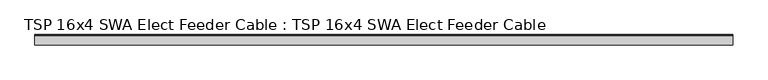
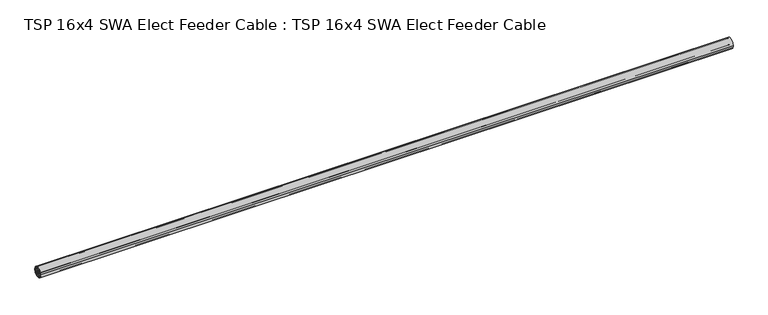
"""IFC4 building model written with IfcOpenShell, lengths in millimetres: proxy geometry, TSP 16x4 SWA Elect Feeder Cable : TSP 16x4 SWA Elect Feeder Cable."""

from ifc_helpers import new_model, si_unit, point, frame, frame_2d, origin, origin_2d, place, context, project, spatial, circle_curve, trimmed, segment, composite_curve, outline, extrude, source, transform, mapped, element, save


def tsp_16x4_swa_elect_feeder_cable_tsp_16x4_swa_elect_feeder_032f6261(model_context):
    return source(origin(), model_context, "Body", "SweptSolid", [
        extrude(outline(composite_curve([segment(trimmed(circle_curve(origin_2d(), 30.0), [point((-30.0, 0.0))], [point((30.0, 0.0))], False, "CARTESIAN"), True, "CONTINUOUS"), segment(trimmed(circle_curve(origin_2d(), 30.0), [point((30.0, 0.0))], [point((-30.0, 0.0))], False, "CARTESIAN"), True, "CONTINUOUS")], self_intersect=False), holes=[composite_curve([segment(trimmed(circle_curve(origin_2d(), 27.0), [point((-27.0, 0.0))], [point((27.0, 0.0))], True, "CARTESIAN"), True, "CONTINUOUS"), segment(trimmed(circle_curve(origin_2d(), 27.0), [point((27.0, 0.0))], [point((-27.0, 0.0))], True, "CARTESIAN"), True, "CONTINUOUS")], self_intersect=False)]), frame((0.0, 0.0, 0.0), z_axis=(1.0, 0.0, 0.0), x_axis=(0.0, 1.0, 0.0)), (0.0, 0.0, 1.0), 4000.0),
        extrude(outline(composite_curve([segment(trimmed(circle_curve(frame_2d((11.691343, 10.1)), 8.0), [point((3.691343, 10.1))], [point((19.691343, 10.1))], False, "CARTESIAN"), True, "CONTINUOUS"), segment(trimmed(circle_curve(frame_2d((11.691343, 10.1)), 8.0), [point((19.691343, 10.1))], [point((3.691343, 10.1))], False, "CARTESIAN"), True, "CONTINUOUS")], self_intersect=False)), frame((0.0, 0.0, 0.0), z_axis=(1.0, 0.0, 0.0), x_axis=(0.0, 1.0, 0.0)), (0.0, 0.0, 1.0), 4000.0),
        extrude(outline(composite_curve([segment(trimmed(circle_curve(frame_2d((-11.691343, 10.1)), 8.0), [point((-19.691343, 10.1))], [point((-3.691343, 10.1))], False, "CARTESIAN"), True, "CONTINUOUS"), segment(trimmed(circle_curve(frame_2d((-11.691343, 10.1)), 8.0), [point((-3.691343, 10.1))], [point((-19.691343, 10.1))], False, "CARTESIAN"), True, "CONTINUOUS")], self_intersect=False)), frame((0.0, 0.0, 0.0), z_axis=(1.0, 0.0, 0.0), x_axis=(0.0, 1.0, 0.0)), (0.0, 0.0, 1.0), 4000.0),
        extrude(outline(composite_curve([segment(trimmed(circle_curve(frame_2d((-11.691343, -10.1)), 8.0), [point((-19.691343, -10.1))], [point((-3.691343, -10.1))], False, "CARTESIAN"), True, "CONTINUOUS"), segment(trimmed(circle_curve(frame_2d((-11.691343, -10.1)), 8.0), [point((-3.691343, -10.1))], [point((-19.691343, -10.1))], False, "CARTESIAN"), True, "CONTINUOUS")], self_intersect=False)), frame((0.0, 0.0, 0.0), z_axis=(1.0, 0.0, 0.0), x_axis=(0.0, 1.0, 0.0)), (0.0, 0.0, 1.0), 4000.0),
        extrude(outline(composite_curve([segment(trimmed(circle_curve(frame_2d((11.691343, -10.1)), 8.0), [point((3.691343, -10.1))], [point((19.691343, -10.1))], False, "CARTESIAN"), True, "CONTINUOUS"), segment(trimmed(circle_curve(frame_2d((11.691343, -10.1)), 8.0), [point((19.691343, -10.1))], [point((3.691343, -10.1))], False, "CARTESIAN"), True, "CONTINUOUS")], self_intersect=False)), frame((0.0, 0.0, 0.0), z_axis=(1.0, 0.0, 0.0), x_axis=(0.0, 1.0, 0.0)), (0.0, 0.0, 1.0), 4000.0),
        extrude(outline(composite_curve([segment(trimmed(circle_curve(origin_2d(), 27.0), [point((27.0, 0.0))], [point((-27.0, 0.0))], False, "CARTESIAN"), True, "CONTINUOUS"), segment(trimmed(circle_curve(origin_2d(), 27.0), [point((-27.0, 0.0))], [point((27.0, 0.0))], False, "CARTESIAN"), True, "CONTINUOUS")], self_intersect=False), holes=[composite_curve([segment(trimmed(circle_curve(frame_2d((-11.691343, 10.1)), 8.0), [point((-3.691343, 10.1))], [point((-19.691343, 10.1))], True, "CARTESIAN"), True, "CONTINUOUS"), segment(trimmed(circle_curve(frame_2d((-11.691343, 10.1)), 8.0), [point((-19.691343, 10.1))], [point((-3.691343, 10.1))], True, "CARTESIAN"), True, "CONTINUOUS")], self_intersect=False), composite_curve([segment(trimmed(circle_curve(frame_2d((11.691343, 10.1)), 8.0), [point((3.691343, 10.1))], [point((19.691343, 10.1))], True, "CARTESIAN"), True, "CONTINUOUS"), segment(trimmed(circle_curve(frame_2d((11.691343, 10.1)), 8.0), [point((19.691343, 10.1))], [point((3.691343, 10.1))], True, "CARTESIAN"), True, "CONTINUOUS")], self_intersect=False), composite_curve([segment(trimmed(circle_curve(frame_2d((-11.691343, -10.15)), 8.0), [point((-19.691343, -10.15))], [point((-3.691343, -10.15))], True, "CARTESIAN"), True, "CONTINUOUS"), segment(trimmed(circle_curve(frame_2d((-11.691343, -10.15)), 8.0), [point((-3.691343, -10.15))], [point((-19.691343, -10.15))], True, "CARTESIAN"), True, "CONTINUOUS")], self_intersect=False), composite_curve([segment(trimmed(circle_curve(frame_2d((11.691343, -10.15)), 8.0), [point((3.691343, -10.15))], [point((19.691343, -10.15))], True, "CARTESIAN"), True, "CONTINUOUS"), segment(trimmed(circle_curve(frame_2d((11.691343, -10.15)), 8.0), [point((19.691343, -10.15))], [point((3.691343, -10.15))], True, "CARTESIAN"), True, "CONTINUOUS")], self_intersect=False)]), frame((0.0, 0.0, 0.0), z_axis=(1.0, 0.0, 0.0), x_axis=(0.0, 1.0, 0.0)), (0.0, 0.0, 1.0), 4000.0),
    ])


if __name__ == "__main__":
    model = new_model("IFC4")
    model_context = context("Model", 3, world=origin())
    ifc_project = project(units=[si_unit("LENGTHUNIT", "METRE", prefix="MILLI")], contexts=[model_context])
    site = spatial("IfcSite", under=ifc_project)
    building = spatial("IfcBuilding", under=site)
    placement = place(None, origin())
    tsp_16x4_swa_elect_feeder_cable_tsp_16x4_swa_elect_feeder_shape = tsp_16x4_swa_elect_feeder_cable_tsp_16x4_swa_elect_feeder_032f6261(model_context)
    element("IfcBuildingElementProxy", 1, Name="TSP 16x4 SWA Elect Feeder Cable : TSP 16x4 SWA Elect Feeder Cable", ObjectType="TSP 16x4 SWA Elect Feeder Cable : TSP 16x4 SWA Elect Feeder Cable", at=placement, inside=building, context=model_context, shape_type="MappedRepresentation", body=[
        mapped(tsp_16x4_swa_elect_feeder_cable_tsp_16x4_swa_elect_feeder_shape, transform((0.0, 0.0, 0.0), x_axis=(1.0, 0.0, 0.0), y_axis=(0.0, 1.0, 0.0), z_axis=(0.0, 0.0, 1.0))),
    ])
    save(model, "model.ifc")

# Revit data of these elements
# Project information
#   Building Name = "BUILDING NAME"
#   Project Issue Date = "YEAR/MONTH/DAY"
#   Project Status = "Project Status"
#   Client Name = "BESPOKE FIRE"
#   Project Address = "Enter address here"
#   Project Name = "REVIT MASTERY LIVE"
#   Project Number = "000"
# Type "TSP 16x4 SWA Elect Feeder Cable : TSP 16x4 SWA Elect Feeder Cable"
#   Model = "TSP_ELECSC164"
#   built-in parameter 1001306 [instance default] = 5.24934 (stored number, unit not read)
#   Cable Length [instance default] = 1600 mm
#   Default Elevation = 0
# Element 1 (IfcBuildingElementProxy, "TSP 16x4 SWA Elect Feeder Cable : TSP 16x4 SWA Elect Feeder Cable")
#   built-in parameter 1001306 = 13.1234 (stored number, unit not read)
#   Cable Length = 4000 mm
#   Materials on its faces: "Cellulose Fill", "Copper", "Laminate, Red, Matte"
# Materials
#   "Cellulose Fill": class "Generic", colour RGB 0 0 0, transparency 0, Description = "Cellulose loose fill", Cost = 0
#   "Copper": class "Metal", colour RGB 0 0 0, transparency 0, Description = "Copper, matte finish", Cost = 0
#   "Laminate, Red, Matte": class "Plastic", colour RGB 255 0 0, transparency 0, Description = "Plastic Laminate - Red, Matte", Cost = 0
